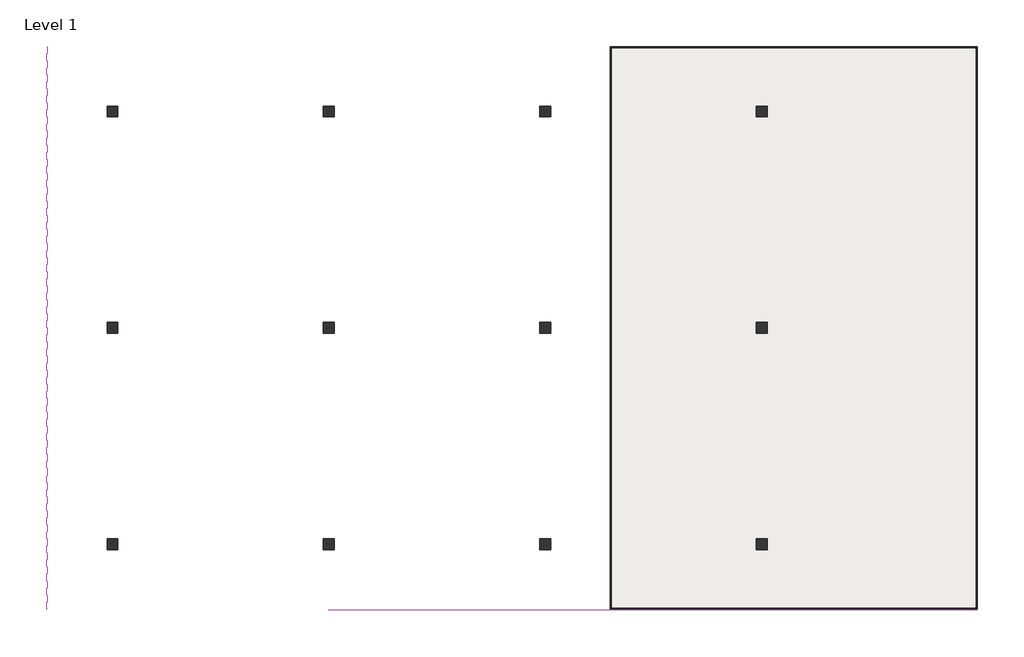
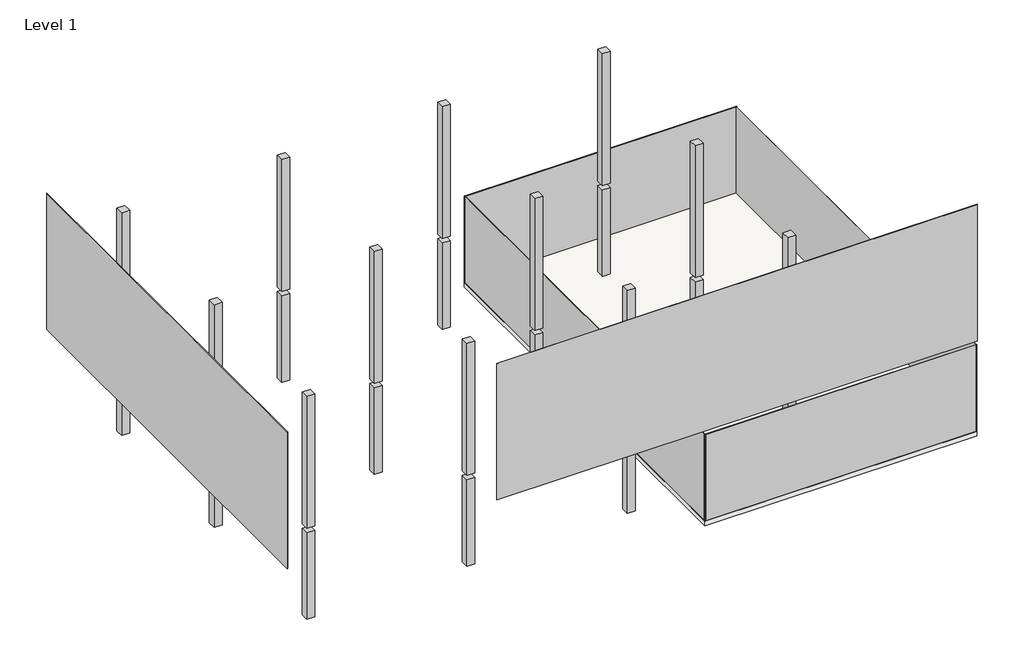
# One storey: 12 columns, 6 plates, 1 slab.
"""IFC4 building model written with IfcOpenShell, lengths in millimetres."""

import ifcopenshell
import ifcopenshell.guid

model = None  # the IFC model being written
_history = None  # IfcOwnerHistory: only IFC2X3 demands one
_inside = {}  # id of a spatial element -> (the spatial element, [elements in it])
_under = {}  # id of a project, library or spatial element -> (it, [spatial elements below it])
_declared = {}  # id of a project -> (the project, [libraries it declares])
_typed = {}  # id of a type object -> (the type object, [elements of that type])
_made_of = {}  # id of a material, layer set ... -> (it, [elements and type objects made of it])


def new_model(schema):
    """Start an empty IFC model of exactly this schema.

    Asked for "IFC4X3", IfcOpenShell would pick the latest addendum, in which some entities
    have other attributes; the version numbers below select the first issue.
    IFC2X3 requires an IfcOwnerHistory on every rooted entity: one is made here for all.
    """
    global model, _history
    if schema == "IFC4X3":
        model = ifcopenshell.file(schema_version=(4, 3, 0, 0))
    else:
        model = ifcopenshell.file(schema=schema)
    _inside.clear()
    _under.clear()
    _declared.clear()
    _typed.clear()
    _made_of.clear()
    _history = None
    if model.schema == "IFC2X3":
        org = make("IfcOrganization", Name="unknown")
        user = make(
            "IfcPersonAndOrganization",
            ThePerson=make("IfcPerson", FamilyName="unknown"),
            TheOrganization=org,
        )
        app = make(
            "IfcApplication",
            ApplicationDeveloper=org,
            Version="unknown",
            ApplicationFullName="unknown",
            ApplicationIdentifier="unknown",
        )
        _history = make(
            "IfcOwnerHistory",
            OwningUser=user,
            OwningApplication=app,
            ChangeAction="ADDED",
            CreationDate=0,
        )
    return model


def make(cls, **values):
    """One entity of the class cls with the attributes given. An attribute that is None is left unset."""
    return model.create_entity(
        cls, **{name: value for name, value in values.items() if value is not None}
    )


def rooted(cls, **values):
    """An entity with a GlobalId (a new one), such as an element, a storey or a relation."""
    return make(cls, GlobalId=ifcopenshell.guid.new(), OwnerHistory=_history, **values)


def si_unit(unit_type, name, prefix=None):
    """IfcSIUnit, for example si_unit("LENGTHUNIT", "METRE", prefix="MILLI")."""
    return make("IfcSIUnit", UnitType=unit_type, Prefix=prefix, Name=name)


def assignment(units):
    """IfcUnitAssignment: the units of a project."""
    return None if units is None else make("IfcUnitAssignment", Units=units)


def point(xyz):
    """IfcCartesianPoint."""
    return None if xyz is None else make("IfcCartesianPoint", Coordinates=xyz)


def direction(xyz):
    """IfcDirection."""
    return None if xyz is None else make("IfcDirection", DirectionRatios=xyz)


def frame(location, z_axis=None, x_axis=None):
    """IfcAxis2Placement3D, a coordinate frame: its origin and axes. An axis left out is left unset."""
    return make(
        "IfcAxis2Placement3D",
        Location=point(location),
        Axis=direction(z_axis),
        RefDirection=direction(x_axis),
    )


def origin():
    """The frame at (0, 0, 0) with its axes left unset."""
    return frame((0.0, 0.0, 0.0))


def origin_with_axes():
    """The frame at (0, 0, 0) with the z axis (0, 0, 1) and the x axis (1, 0, 0) written out."""
    return frame((0.0, 0.0, 0.0), z_axis=(0.0, 0.0, 1.0), x_axis=(1.0, 0.0, 0.0))


def place(relative_to, where):
    """IfcLocalPlacement: puts the frame where relative to a parent placement (None: the world)."""
    return make(
        "IfcLocalPlacement", PlacementRelTo=relative_to, RelativePlacement=where
    )


def context(
    kind, dimensions, precision=None, world=None, true_north=None, identifier=None
):
    """IfcGeometricRepresentationContext, for example the 3D "Model" context."""
    return make(
        "IfcGeometricRepresentationContext",
        ContextIdentifier=identifier,
        ContextType=kind,
        CoordinateSpaceDimension=dimensions,
        Precision=precision,
        WorldCoordinateSystem=world,
        TrueNorth=true_north,
    )


def project(units=None, contexts=None):
    """IfcProject with its units and contexts."""
    return rooted(
        "IfcProject",
        Name="project",
        RepresentationContexts=contexts,
        UnitsInContext=assignment(units),
    )


def spatial(cls, under=None, at=None, **own):
    """A site, building, storey or space (cls), placed at a placement, below another one or the project."""
    s = rooted(cls, ObjectPlacement=at, **own)
    if under is not None:
        _under.setdefault(under.id(), (under, []))[1].append(s)
    return s


def polyline(points):
    """IfcPolyline through the points."""
    return make("IfcPolyline", Points=[point(p) for p in points])


def outline(outer, holes=None, kind="AREA"):
    """IfcArbitraryClosedProfileDef: a profile drawn as a closed curve; with holes, ...WithVoids."""
    if holes is None:
        return make("IfcArbitraryClosedProfileDef", ProfileType=kind, OuterCurve=outer)
    return make(
        "IfcArbitraryProfileDefWithVoids",
        ProfileType=kind,
        OuterCurve=outer,
        InnerCurves=holes,
    )


def extrude(swept, where, along, depth):
    """IfcExtrudedAreaSolid: the profile swept, set in the frame where, extruded along a direction by depth."""
    return make(
        "IfcExtrudedAreaSolid",
        SweptArea=swept,
        Position=where,
        ExtrudedDirection=direction(along),
        Depth=depth,
    )


def shape(context_of_items, identifier, shape_type, items):
    """IfcShapeRepresentation: the items that make up one representation, for example the "Body"."""
    return make(
        "IfcShapeRepresentation",
        ContextOfItems=context_of_items,
        RepresentationIdentifier=identifier,
        RepresentationType=shape_type,
        Items=items,
    )


def source(mapping_origin, context_of_items, identifier, shape_type, items):
    """IfcRepresentationMap: a shape defined once, which mapped items show again and again."""
    return make(
        "IfcRepresentationMap",
        MappingOrigin=mapping_origin,
        MappedRepresentation=shape(context_of_items, identifier, shape_type, items),
    )


def transform(
    local_origin,
    x_axis=None,
    y_axis=None,
    z_axis=None,
    scale=None,
    scale2=None,
    scale3=None,
    uniform=True,
):
    """IfcCartesianTransformationOperator3D, or its non-uniform kind. x_axis, y_axis, z_axis: its Axis1, 2, 3."""
    if uniform:
        return make(
            "IfcCartesianTransformationOperator3D",
            Axis1=direction(x_axis),
            Axis2=direction(y_axis),
            LocalOrigin=point(local_origin),
            Scale=scale,
            Axis3=direction(z_axis),
        )
    return make(
        "IfcCartesianTransformationOperator3DnonUniform",
        Axis1=direction(x_axis),
        Axis2=direction(y_axis),
        LocalOrigin=point(local_origin),
        Scale=scale,
        Axis3=direction(z_axis),
        Scale2=scale2,
        Scale3=scale3,
    )


def mapped(mapping_source, mapping_target):
    """IfcMappedItem: shows the shape of a source again, moved by a transform."""
    return make(
        "IfcMappedItem", MappingSource=mapping_source, MappingTarget=mapping_target
    )


def made_of(thing, what):
    """Note that an element or type object is made of a material, layer set ...; save() writes the relation."""
    if what is not None:
        _made_of.setdefault(what.id(), (what, []))[1].append(thing)
    return thing


def element(
    cls,
    number,
    at=None,
    inside=None,
    cuts=None,
    type_object=None,
    material=None,
    context=None,
    identifier="Body",
    shape_type=None,
    held_by="IfcProductDefinitionShape",
    body=None,
    shapes=None,
    **own,
):
    """One element of the class cls, such as IfcWall. Its Tag is "e" and its number.

    at: its placement. inside: the storey or other place that contains it. cuts: it is an
    opening in that element (IfcRelVoidsElement). A single representation is given by context,
    identifier, shape_type and body (its items); several are given by shapes. held_by: the class
    of the entity that holds the representations. save() writes the other relations.
    """
    e = rooted(cls, Tag="e%d" % number, ObjectPlacement=at, **own)
    if body is not None:
        shapes = [shape(context, identifier, shape_type, body)]
    if shapes is not None:
        e.Representation = make(held_by, Representations=shapes)
    if inside is not None:
        _inside.setdefault(inside.id(), (inside, []))[1].append(e)
    if cuts is not None:
        rooted(
            "IfcRelVoidsElement", RelatingBuildingElement=cuts, RelatedOpeningElement=e
        )
    if type_object is not None:
        _typed.setdefault(type_object.id(), (type_object, []))[1].append(e)
    return made_of(e, material)


def aggregate(whole, parts):
    """IfcRelAggregates: a whole, such as a stair, and the parts it consists of."""
    return rooted("IfcRelAggregates", RelatingObject=whole, RelatedObjects=parts)


def save(model, path):
    """Write the relations noted so far, then the file.

    IfcRelAggregates (storeys below a building ...), IfcRelContainedInSpatialStructure (elements
    in a storey), IfcRelDefinesByType, IfcRelAssociatesMaterial and IfcRelDeclares: one each for
    every whole, place, type object, material and project.
    """
    for whole, parts in _under.values():
        aggregate(whole, parts)
    for where, things in _inside.values():
        rooted(
            "IfcRelContainedInSpatialStructure",
            RelatedElements=things,
            RelatingStructure=where,
        )
    for kind, things in _typed.values():
        rooted("IfcRelDefinesByType", RelatedObjects=things, RelatingType=kind)
    for what, things in _made_of.values():
        rooted("IfcRelAssociatesMaterial", RelatedObjects=things, RelatingMaterial=what)
    for by, libraries in _declared.values():
        rooted("IfcRelDeclares", RelatingContext=by, RelatedDefinitions=libraries)
    model.write(path)


def system_panel_glazed_8c8fe697(model_context):
    return source(origin(), model_context, "Body", "SweptSolid", [
        extrude(outline(polyline([(13000.0, 24.5), (-13000.0, 24.5), (-13000.0, 49.5), (13000.0, 49.5), (13000.0, 24.5)])), origin_with_axes(), (0.0, 0.0, 1.0), 5700.0),
    ])


def system_panel_glazed_08161773(model_context):
    return source(origin(), model_context, "Body", "SweptSolid", [
        extrude(outline(polyline([(8487.75, 24.5), (-8487.75, 24.5), (-8487.75, 49.5), (8487.75, 49.5), (8487.75, 24.5)])), origin_with_axes(), (0.0, 0.0, 1.0), 5700.0),
    ])


def system_panel_glazed_8cf960c6(model_context):
    return source(origin(), model_context, "Body", "SweptSolid", [
        extrude(outline(polyline([(13000.0, 24.5), (-13000.0, 24.5), (-13000.0, 49.5), (13000.0, 49.5), (13000.0, 24.5)])), origin_with_axes(), (0.0, 0.0, 1.0), 9000.0),
    ])


def system_panel_glazed_15d59c4f(model_context):
    return source(origin(), model_context, "Body", "SweptSolid", [
        extrude(outline(polyline([(14987.75, 24.5), (-14987.75, 24.5), (-14987.75, 49.5), (14987.75, 49.5), (14987.75, 24.5)])), origin_with_axes(), (0.0, 0.0, 1.0), 9000.0),
    ])


model = new_model("IFC4")

# Units and contexts
model_context = context("Model", 3, world=origin())
ifc_project = project(units=[si_unit("LENGTHUNIT", "METRE", prefix="MILLI")], contexts=[model_context])

# Site, building, storey
site = spatial("IfcSite", under=ifc_project)
building = spatial("IfcBuilding", under=site)
storey = spatial("IfcBuildingStorey", under=building, Name="Level 1", Elevation=0.0)

# Columns
placement = place(None, origin())
element("IfcColumn", 1, ObjectType="콘크리트-정사각형-기둥 : 500 x 500", at=placement, inside=storey, context=model_context, shape_type="SweptSolid", body=[
    extrude(outline(polyline([(-3482.0028633, 13248.757723), (-3482.0028633, 12748.757723), (-3982.0028633, 12748.757723), (-3982.0028633, 13248.757723), (-3482.0028633, 13248.757723)])), origin_with_axes(), (0.0, 0.0, 1.0), 5700.0),
    extrude(outline(polyline([(-3482.0028633, 13248.757723), (-3482.0028633, 12748.757723), (-3982.0028633, 12748.757723), (-3982.0028633, 13248.757723), (-3482.0028633, 13248.757723)])), frame((0.0, 0.0, 6000.0), z_axis=(0.0, 0.0, 1.0), x_axis=(1.0, 0.0, 0.0)), (0.0, 0.0, 1.0), 8700.0),
])
element("IfcColumn", 2, ObjectType="콘크리트-정사각형-기둥 : 500 x 500", at=placement, inside=storey, context=model_context, shape_type="SweptSolid", body=[
    extrude(outline(polyline([(-3482.0028633, 3248.757723), (-3482.0028633, 2748.757723), (-3982.0028633, 2748.757723), (-3982.0028633, 3248.757723), (-3482.0028633, 3248.757723)])), origin_with_axes(), (0.0, 0.0, 1.0), 5700.0),
    extrude(outline(polyline([(-3482.0028633, 3248.757723), (-3482.0028633, 2748.757723), (-3982.0028633, 2748.757723), (-3982.0028633, 3248.757723), (-3482.0028633, 3248.757723)])), frame((0.0, 0.0, 6000.0), z_axis=(0.0, 0.0, 1.0), x_axis=(1.0, 0.0, 0.0)), (0.0, 0.0, 1.0), 8700.0),
])
element("IfcColumn", 3, ObjectType="콘크리트-정사각형-기둥 : 500 x 500", at=placement, inside=storey, context=model_context, shape_type="SweptSolid", body=[
    extrude(outline(polyline([(-3482.0028633, -6751.242277), (-3482.0028633, -7251.242277), (-3982.0028633, -7251.242277), (-3982.0028633, -6751.242277), (-3482.0028633, -6751.242277)])), origin_with_axes(), (0.0, 0.0, 1.0), 5700.0),
    extrude(outline(polyline([(-3482.0028633, -6751.242277), (-3482.0028633, -7251.242277), (-3982.0028633, -7251.242277), (-3982.0028633, -6751.242277), (-3482.0028633, -6751.242277)])), frame((0.0, 0.0, 6000.0), z_axis=(0.0, 0.0, 1.0), x_axis=(1.0, 0.0, 0.0)), (0.0, 0.0, 1.0), 8700.0),
])
element("IfcColumn", 4, ObjectType="콘크리트-정사각형-기둥 : 500 x 500", at=placement, inside=storey, context=model_context, shape_type="SweptSolid", body=[
    extrude(outline(polyline([(6517.9971367, 13248.757723), (6517.9971367, 12748.757723), (6017.9971367, 12748.757723), (6017.9971367, 13248.757723), (6517.9971367, 13248.757723)])), origin_with_axes(), (0.0, 0.0, 1.0), 5700.0),
    extrude(outline(polyline([(6517.9971367, 13248.757723), (6517.9971367, 12748.757723), (6017.9971367, 12748.757723), (6017.9971367, 13248.757723), (6517.9971367, 13248.757723)])), frame((0.0, 0.0, 6000.0), z_axis=(0.0, 0.0, 1.0), x_axis=(1.0, 0.0, 0.0)), (0.0, 0.0, 1.0), 8700.0),
])
element("IfcColumn", 5, ObjectType="콘크리트-정사각형-기둥 : 500 x 500", at=placement, inside=storey, context=model_context, shape_type="SweptSolid", body=[
    extrude(outline(polyline([(6517.9971367, 3248.757723), (6517.9971367, 2748.757723), (6017.9971367, 2748.757723), (6017.9971367, 3248.757723), (6517.9971367, 3248.757723)])), origin_with_axes(), (0.0, 0.0, 1.0), 5700.0),
    extrude(outline(polyline([(6517.9971367, 3248.757723), (6517.9971367, 2748.757723), (6017.9971367, 2748.757723), (6017.9971367, 3248.757723), (6517.9971367, 3248.757723)])), frame((0.0, 0.0, 6000.0), z_axis=(0.0, 0.0, 1.0), x_axis=(1.0, 0.0, 0.0)), (0.0, 0.0, 1.0), 8700.0),
])
element("IfcColumn", 6, ObjectType="콘크리트-정사각형-기둥 : 500 x 500", at=placement, inside=storey, context=model_context, shape_type="SweptSolid", body=[
    extrude(outline(polyline([(6517.9971367, -6751.242277), (6517.9971367, -7251.242277), (6017.9971367, -7251.242277), (6017.9971367, -6751.242277), (6517.9971367, -6751.242277)])), origin_with_axes(), (0.0, 0.0, 1.0), 5700.0),
    extrude(outline(polyline([(6517.9971367, -6751.242277), (6517.9971367, -7251.242277), (6017.9971367, -7251.242277), (6017.9971367, -6751.242277), (6517.9971367, -6751.242277)])), frame((0.0, 0.0, 6000.0), z_axis=(0.0, 0.0, 1.0), x_axis=(1.0, 0.0, 0.0)), (0.0, 0.0, 1.0), 8700.0),
])
element("IfcColumn", 7, ObjectType="콘크리트-정사각형-기둥 : 500 x 500", at=placement, inside=storey, context=model_context, shape_type="SweptSolid", body=[
    extrude(outline(polyline([(16517.9971367, 13248.757723), (16517.9971367, 12748.757723), (16017.9971367, 12748.757723), (16017.9971367, 13248.757723), (16517.9971367, 13248.757723)])), origin_with_axes(), (0.0, 0.0, 1.0), 5700.0),
    extrude(outline(polyline([(16517.9971367, 13248.757723), (16517.9971367, 12748.757723), (16017.9971367, 12748.757723), (16017.9971367, 13248.757723), (16517.9971367, 13248.757723)])), frame((0.0, 0.0, 6000.0), z_axis=(0.0, 0.0, 1.0), x_axis=(1.0, 0.0, 0.0)), (0.0, 0.0, 1.0), 8700.0),
])
element("IfcColumn", 8, ObjectType="콘크리트-정사각형-기둥 : 500 x 500", at=placement, inside=storey, context=model_context, shape_type="SweptSolid", body=[
    extrude(outline(polyline([(16517.9971367, 3248.757723), (16517.9971367, 2748.757723), (16017.9971367, 2748.757723), (16017.9971367, 3248.757723), (16517.9971367, 3248.757723)])), origin_with_axes(), (0.0, 0.0, 1.0), 5700.0),
    extrude(outline(polyline([(16517.9971367, 3248.757723), (16517.9971367, 2748.757723), (16017.9971367, 2748.757723), (16017.9971367, 3248.757723), (16517.9971367, 3248.757723)])), frame((0.0, 0.0, 6000.0), z_axis=(0.0, 0.0, 1.0), x_axis=(1.0, 0.0, 0.0)), (0.0, 0.0, 1.0), 8700.0),
])
element("IfcColumn", 9, ObjectType="콘크리트-정사각형-기둥 : 500 x 500", at=placement, inside=storey, context=model_context, shape_type="SweptSolid", body=[
    extrude(outline(polyline([(16517.9971367, -6751.242277), (16517.9971367, -7251.242277), (16017.9971367, -7251.242277), (16017.9971367, -6751.242277), (16517.9971367, -6751.242277)])), origin_with_axes(), (0.0, 0.0, 1.0), 5700.0),
    extrude(outline(polyline([(16517.9971367, -6751.242277), (16517.9971367, -7251.242277), (16017.9971367, -7251.242277), (16017.9971367, -6751.242277), (16517.9971367, -6751.242277)])), frame((0.0, 0.0, 6000.0), z_axis=(0.0, 0.0, 1.0), x_axis=(1.0, 0.0, 0.0)), (0.0, 0.0, 1.0), 8700.0),
])
element("IfcColumn", 10, ObjectType="콘크리트-정사각형-기둥 : 500 x 500", at=placement, inside=storey, context=model_context, shape_type="SweptSolid", body=[
    extrude(outline(polyline([(26517.9971367, 13248.757723), (26517.9971367, 12748.757723), (26017.9971367, 12748.757723), (26017.9971367, 13248.757723), (26517.9971367, 13248.757723)])), origin_with_axes(), (0.0, 0.0, 1.0), 5700.0),
    extrude(outline(polyline([(26517.9971367, 13248.757723), (26517.9971367, 12748.757723), (26017.9971367, 12748.757723), (26017.9971367, 13248.757723), (26517.9971367, 13248.757723)])), frame((0.0, 0.0, 6000.0), z_axis=(0.0, 0.0, 1.0), x_axis=(1.0, 0.0, 0.0)), (0.0, 0.0, 1.0), 8700.0),
])
element("IfcColumn", 11, ObjectType="콘크리트-정사각형-기둥 : 500 x 500", at=placement, inside=storey, context=model_context, shape_type="SweptSolid", body=[
    extrude(outline(polyline([(26517.9971367, 3248.757723), (26517.9971367, 2748.757723), (26017.9971367, 2748.757723), (26017.9971367, 3248.757723), (26517.9971367, 3248.757723)])), origin_with_axes(), (0.0, 0.0, 1.0), 5700.0),
    extrude(outline(polyline([(26517.9971367, 3248.757723), (26517.9971367, 2748.757723), (26017.9971367, 2748.757723), (26017.9971367, 3248.757723), (26517.9971367, 3248.757723)])), frame((0.0, 0.0, 6000.0), z_axis=(0.0, 0.0, 1.0), x_axis=(1.0, 0.0, 0.0)), (0.0, 0.0, 1.0), 8700.0),
])
element("IfcColumn", 12, ObjectType="콘크리트-정사각형-기둥 : 500 x 500", at=placement, inside=storey, context=model_context, shape_type="SweptSolid", body=[
    extrude(outline(polyline([(26517.9971367, -6751.242277), (26517.9971367, -7251.242277), (26017.9971367, -7251.242277), (26017.9971367, -6751.242277), (26517.9971367, -6751.242277)])), origin_with_axes(), (0.0, 0.0, 1.0), 5700.0),
    extrude(outline(polyline([(26517.9971367, -6751.242277), (26517.9971367, -7251.242277), (26017.9971367, -7251.242277), (26017.9971367, -6751.242277), (26517.9971367, -6751.242277)])), frame((0.0, 0.0, 6000.0), z_axis=(0.0, 0.0, 1.0), x_axis=(1.0, 0.0, 0.0)), (0.0, 0.0, 1.0), 8700.0),
])

# Plates
system_panel_glazed_shape = system_panel_glazed_8c8fe697(model_context)
element("IfcPlate", 13, ObjectType="System Panel : Glazed", at=placement, inside=storey, context=model_context, shape_type="MappedRepresentation", body=[
    mapped(system_panel_glazed_shape, transform((36243.4971367, 2998.757723, 0.0), x_axis=(0.0, 1.0, 0.0), y_axis=(-1.0, 0.0, 0.0), z_axis=(0.0, 0.0, 1.0))),
])
element("IfcPlate", 14, ObjectType="System Panel : Glazed", at=placement, inside=storey, context=model_context, shape_type="MappedRepresentation", body=[
    mapped(system_panel_glazed_shape, transform((19267.9971367, 2998.757723, 0.0), x_axis=(0.0, -1.0, 0.0), y_axis=(1.0, 0.0, 0.0), z_axis=(0.0, 0.0, 1.0))),
])
system_panel_glazed_2_shape = system_panel_glazed_08161773(model_context)
element("IfcPlate", 15, ObjectType="System Panel : Glazed", at=placement, inside=storey, context=model_context, shape_type="MappedRepresentation", body=[
    mapped(system_panel_glazed_2_shape, transform((27755.7471367, 15998.757723, 0.0), x_axis=(-1.0, 0.0, 0.0), y_axis=(0.0, -1.0, 0.0), z_axis=(0.0, 0.0, 1.0))),
])
element("IfcPlate", 16, ObjectType="System Panel : Glazed", at=placement, inside=storey, context=model_context, shape_type="MappedRepresentation", body=[
    mapped(system_panel_glazed_2_shape, transform((27755.7471367, -10001.242277, 0.0), x_axis=(1.0, 0.0, 0.0), y_axis=(0.0, 1.0, 0.0), z_axis=(0.0, 0.0, 1.0))),
])
system_panel_glazed_3_shape = system_panel_glazed_8cf960c6(model_context)
element("IfcPlate", 17, ObjectType="System Panel : Glazed", at=placement, inside=storey, context=model_context, shape_type="MappedRepresentation", body=[
    mapped(system_panel_glazed_3_shape, transform((-6732.0028633, 2998.757723, 6000.0), x_axis=(0.0, 1.0, 0.0), y_axis=(-1.0, 0.0, 0.0), z_axis=(0.0, 0.0, 1.0))),
])
system_panel_glazed_4_shape = system_panel_glazed_15d59c4f(model_context)
element("IfcPlate", 18, ObjectType="System Panel : Glazed", at=placement, inside=storey, context=model_context, shape_type="MappedRepresentation", body=[
    mapped(system_panel_glazed_4_shape, transform((21255.7471367, -10001.242277, 6000.0), x_axis=(-1.0, 0.0, 0.0), y_axis=(0.0, -1.0, 0.0), z_axis=(0.0, 0.0, 1.0))),
])

# Slab
element("IfcSlab", 19, ObjectType="Generic 300mm", at=placement, inside=storey, context=model_context, shape_type="SweptSolid", body=[
    extrude(outline(polyline([(19267.9971367, 15998.757723), (36243.4971367, 15998.757723), (36243.4971367, -10001.242277), (19267.9971367, -10001.242277), (19267.9971367, 15998.757723)])), frame((0.0, 0.0, -300.0), z_axis=(0.0, 0.0, 1.0), x_axis=(1.0, 0.0, 0.0)), (0.0, 0.0, 1.0), 300.0),
])

save(model, "model.ifc")

# Revit data of these elements
# Project information
#   Project Issue Date = "Issue Date"
#   Project Status = "Project Status"
#   Client Name = "Owner"
#   Project Address = "Enter address here"
#   Project Name = "Project Name"
#   Project Number = "Project Number"
#   Document GUID = "c2a387e2-990c-40c9-8e77-3791c5d4ece9"
# Grids (mm)
#   "1": line (-6732.003, -17149.184) -> (-6732.003, 20035.144)
#   "2": line (-3732.003, -17149.184) -> (-3732.003, 20035.144)
#   "3": line (6267.997, -17149.184) -> (6267.997, 20035.144)
#   "4": line (16267.997, -17149.184) -> (16267.997, 20035.144)
#   "5": line (26267.997, -17149.184) -> (26267.997, 20035.144)
#   "6": line (36243.497, -17149.184) -> (36243.497, 20035.144)
#   "A": line (42039.58, 15998.758) -> (-12000.946, 15998.758)
#   "B": line (42039.58, 12998.758) -> (-12000.946, 12998.758)
#   "C": line (42039.58, 2998.758) -> (-12000.946, 2998.758)
#   "D": line (42039.58, -7001.242) -> (-12000.946, -7001.242)
#   "E": line (42039.58, -10001.242) -> (-12000.946, -10001.242)
# Type "콘크리트-정사각형-기둥 : 500 x 500"
#   b = 0.500 m
#   Structural Material [instance default] = 콘크리트 - 현장타설 콘크리트
# Type "Generic 300mm"
#   Function = 0
#   Layers, outside or top first: 0.300 m no material (function 1)
# Elements 1, 2, 3, 4, 5, 6, 7, 8, 9, 10, 11, 12 (IfcColumn, "콘크리트-정사각형-기둥 : 500 x 500")
#   Comments = ""
#   Structural Material = 콘크리트 - 현장타설 콘크리트
#   Phase Created = New Construction
#   Materials on its faces: "콘크리트 - 현장타설 콘크리트"
# Elements 13, 14, 15, 16, 17, 18 (IfcPlate, "System Panel : Glazed")
#   Phase Created = New Construction
#   Materials on its faces: "Glass"
# Element 19 (IfcSlab, "Generic 300mm")
#   built-in parameter 1001955 = 3.14159 (stored number, unit not read)
#   Height Offset From Level = 0.000 m
#   Phase Created = New Construction
#   Materials on its faces: "Default Floor"
# Materials
#   "콘크리트 - 현장타설 콘크리트": class "콘크리트", colour RGB 192 192 192, transparency 0
#   "Glass": class "Glass", colour RGB 0 128 192, transparency 0.9
#   "Default Floor": class "Miscellaneous", colour RGB 127 127 127, transparency 0
